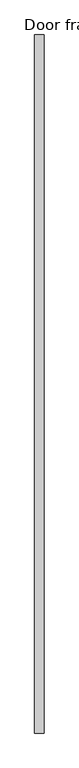
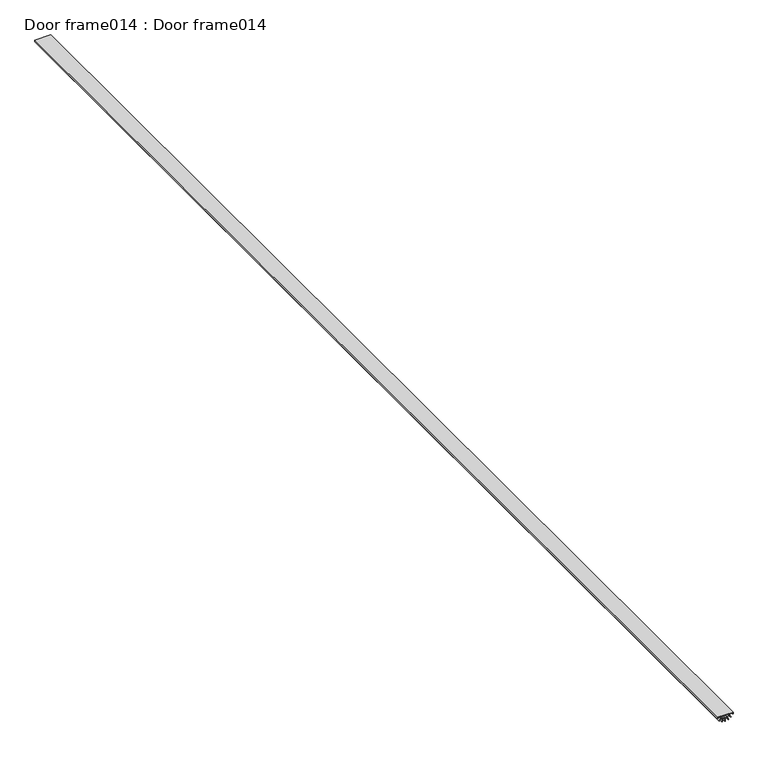
"""IFC4 building model written with IfcOpenShell, lengths in millimetres: proxy geometry, Door frame014 : Door frame014."""

from ifc_helpers import new_model, si_unit, frame, origin, place, context, project, spatial, polyline, outline, extrude, source, transform, mapped, element, save


def door_frame014_door_frame014_1e3dbea9(model_context):
    return source(origin(), model_context, "Body", "SweptSolid", [
        extrude(outline(polyline([(36578.3756733, 15524.8710245), (36578.3756733, 15525.6647745), (36583.8229098, 15525.6647745), (36584.304169, 15528.4194862), (36579.1830903, 15530.2833952), (36579.4545674, 15531.0292768), (36584.573299, 15529.166222), (36585.9800182, 15531.6205482), (36581.8052868, 15535.1235857), (36582.3155014, 15535.731632), (36586.4883159, 15532.2302029), (36588.5541303, 15533.9941318), (36588.5541303, 15536.9862907), (36587.284361, 15536.9862907), (36587.284361, 15538.6848615), (36589.8546103, 15538.6848615), (36589.8546103, 15511.5429442), (36587.284361, 15511.5429442), (36587.284361, 15513.5495083), (36588.5541303, 15513.5495083), (36588.5541303, 15516.5416672), (36586.5323252, 15518.2570371), (36582.3575787, 15514.7540195), (36581.8473669, 15515.362068), (36586.0201974, 15518.8634779), (36584.5980367, 15521.3089171), (36579.4769756, 15519.4449702), (36579.2054928, 15520.1908496), (36584.3242102, 15522.0539435), (36583.8229098, 15524.8710245), (36578.3756733, 15524.8710245)]), holes=[polyline([(36588.5541303, 15532.8858954), (36586.6136518, 15530.8738124), (36585.2069325, 15528.4194862), (36584.7256733, 15525.6647745), (36584.7256733, 15524.8710245), (36585.2269736, 15522.0539435), (36586.6491343, 15519.6085043), (36588.5541303, 15517.6499036), (36588.5541303, 15532.8858954)])]), frame((0.0, -1052.8906567, 0.0), z_axis=(0.0, 1.0, 0.0), x_axis=(0.0, 0.0, 1.0)), (0.0, 0.0, 1.0), 1999.85),
    ])


if __name__ == "__main__":
    model = new_model("IFC4")
    model_context = context("Model", 3, world=origin())
    ifc_project = project(units=[si_unit("LENGTHUNIT", "METRE", prefix="MILLI")], contexts=[model_context])
    site = spatial("IfcSite", under=ifc_project)
    building = spatial("IfcBuilding", under=site)
    placement = place(None, origin())
    door_frame014_door_frame014_shape = door_frame014_door_frame014_1e3dbea9(model_context)
    element("IfcBuildingElementProxy", 1, Name="Door frame014 : Door frame014", ObjectType="Door frame014 : Door frame014", at=placement, inside=building, context=model_context, shape_type="MappedRepresentation", body=[
        mapped(door_frame014_door_frame014_shape, transform((0.0, 0.0, 0.0), x_axis=(1.0, 0.0, 0.0), y_axis=(0.0, 1.0, 0.0), z_axis=(0.0, 0.0, 1.0))),
    ])
    save(model, "model.ifc")

# Revit data of these elements
# Type "Door frame014 : Door frame014"
#   NameOverride = "Door frame014"
# Element 1 (IfcBuildingElementProxy, "Door frame014 : Door frame014")
#   Materials on its faces: "WEATHERSTRIPPING SWEEP"
# Materials
#   "WEATHERSTRIPPING SWEEP": class "Wood", colour RGB 212 179 113, transparency 0, Description = "Plywood, sheathing grade", Cost = 0
